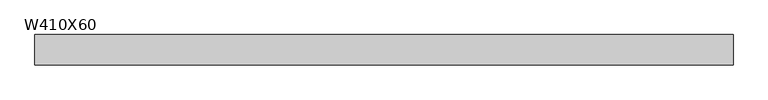
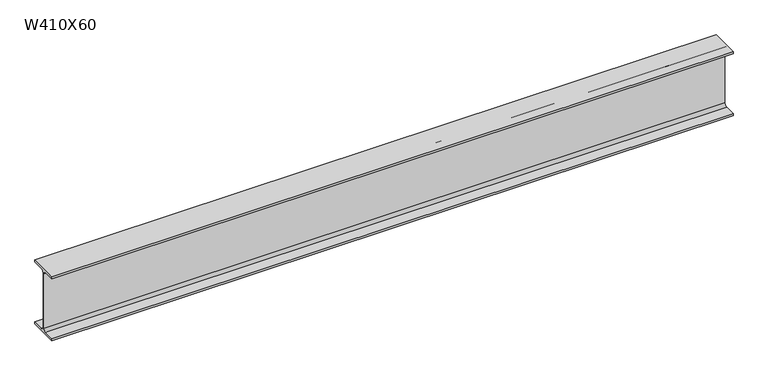
"""IFC4 building model written with IfcOpenShell, lengths in millimetres: beam geometry, M_W-Wide Flange : W410X60."""

from ifc_helpers import new_model, si_unit, point, frame, frame_2d, origin, place, context, project, spatial, polyline, circle_curve, trimmed, segment, composite_curve, outline, extrude, source, transform, mapped, element, save


def w410x60_ca7ba955(model_context):
    return source(origin(), model_context, "Body", "SweptSolid", [
        extrude(outline(composite_curve([segment(polyline([(89.0, -190.7), (89.0, -203.5), (-89.0, -203.5), (-89.0, -190.7), (-21.05, -190.7)]), True, "CONTINUOUS"), segment(trimmed(circle_curve(frame_2d((-21.05, -173.5)), 17.2), [point((-21.05, -190.7))], [point((-3.85, -173.5))], True, "CARTESIAN"), True, "CONTINUOUS"), segment(polyline([(-3.85, -173.5), (-3.85, 173.5)]), True, "CONTINUOUS"), segment(trimmed(circle_curve(frame_2d((-21.05, 173.5)), 17.2), [point((-3.85, 173.5))], [point((-21.05, 190.7))], True, "CARTESIAN"), True, "CONTINUOUS"), segment(polyline([(-21.05, 190.7), (-89.0, 190.7), (-89.0, 203.5), (89.0, 203.5), (89.0, 190.7), (21.05, 190.7)]), True, "CONTINUOUS"), segment(trimmed(circle_curve(frame_2d((21.05, 173.5)), 17.2), [point((21.05, 190.7))], [point((3.85, 173.5))], True, "CARTESIAN"), True, "CONTINUOUS"), segment(polyline([(3.85, 173.5), (3.85, -173.5)]), True, "CONTINUOUS"), segment(trimmed(circle_curve(frame_2d((21.05, -173.5)), 17.2), [point((3.85, -173.5))], [point((21.05, -190.7))], True, "CARTESIAN"), True, "CONTINUOUS"), segment(polyline([(21.05, -190.7), (89.0, -190.7)]), True, "CONTINUOUS")], self_intersect=False)), frame((-2050.0, 0.0, 0.0), z_axis=(1.0, 0.0, 0.0), x_axis=(0.0, 1.0, 0.0)), (0.0, 0.0, 1.0), 4100.0),
    ])


if __name__ == "__main__":
    model = new_model("IFC4")
    model_context = context("Model", 3, world=origin())
    ifc_project = project(units=[si_unit("LENGTHUNIT", "METRE", prefix="MILLI")], contexts=[model_context])
    site = spatial("IfcSite", under=ifc_project)
    building = spatial("IfcBuilding", under=site)
    placement = place(None, origin())
    w410x60_shape = w410x60_ca7ba955(model_context)
    element("IfcBeam", 1, ObjectType="M_W-Wide Flange : W410X60", at=placement, inside=building, context=model_context, shape_type="MappedRepresentation", body=[
        mapped(w410x60_shape, transform((0.0, 0.0, 0.0), x_axis=(1.0, 0.0, 0.0), y_axis=(0.0, 1.0, 0.0), z_axis=(0.0, 0.0, 1.0))),
    ])
    save(model, "model.ifc")

# Revit data of these elements
# Type "M_W-Wide Flange : W410X60"
#   Manufacturer = "Manufacturer"
#   AccessibilityPerformance = "AccessibilityPerformance"
#   CodePerformance = "CodePerformance"
#   Color = "Color"
#   Constituents = "Constituents"
#   Features = "Features"
#   Finish = "Finish"
#   Grade = "Grade"
#   Material = "Material"
#   ModelReference = "ModelReference"
#   NominalHeight = "NominalHeight"
#   NominalLength = "NominalLength"
#   NominalWidth = "NominalWidth"
#   ProductionYear = "ProductionYear"
#   Reference = "Reference"
#   Shape = "Shape"
#   Size = "Size"
#   SustainabilityPerformance = "SustainabilityPerformance"
#   WarrantyDescription = "WarrantyDescription"
#   WarrantyDurationLabor = "WarrantyDurationLabor"
#   WarrantyDurationParts = "WarrantyDurationParts"
#   WarrantyGuarantorLabor = "WarrantyGuarantorLabor"
#   WarrantyGuarantorParts = "WarrantyGuarantorParts"
#   ExpectedLife = "ExpectedLife"
#   ReplacementCost = "ReplacementCost"
#   AssetAccountingType = "FIXED"
#   ModelLabel = "ModelLabel"
#   W = 0.58
#   Start Extension Calculation [instance default] = 3.000 m
#   Start Extension [instance default] = -0.0127 m
#   End Extension Calculation [instance default] = 3.000 m
#   End Extension [instance default] = -0.0127 m
#   Length [instance default] = 1.524 m
#   bf = 0.178 m
#   d = 0.407 m
#   k = 0.030 m
#   kr = 0.0172 m
#   tf = 0.0128 m
#   tw = 0.0077 m
#   A = 0.0076 m²
#   Structural Material [instance default] = Metal - Steel - 345 MPa
#   Assembly Code = ""
# Element 1 (IfcBeam, "M_W-Wide Flange : W410X60")
#   Materials on its faces: "Metal - Steel - 345 MPa"
# Materials
#   "Metal - Steel - 345 MPa": class "Metal", colour RGB 247 247 247, transparency 0
